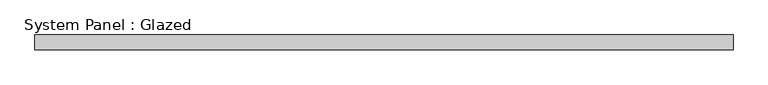
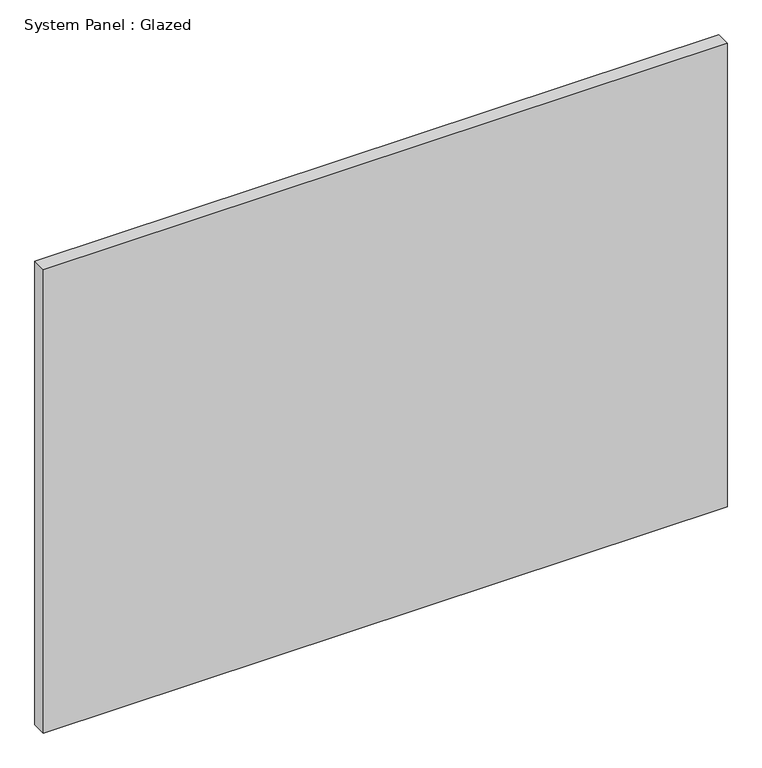
"""IFC4 building model written with IfcOpenShell, lengths in millimetres: plate geometry, System Panel : Glazed."""

from ifc_helpers import new_model, si_unit, origin, origin_with_axes, place, context, project, spatial, polyline, outline, extrude, source, transform, mapped, element, save


def system_panel_glazed_00a161e3(model_context):
    return source(origin(), model_context, "Body", "SweptSolid", [
        extrude(outline(polyline([(593.725, 19.05), (-593.725, 19.05), (-593.725, 44.45), (593.725, 44.45), (593.725, 19.05)])), origin_with_axes(), (0.0, 0.0, 1.0), 850.9),
    ])


if __name__ == "__main__":
    model = new_model("IFC4")
    model_context = context("Model", 3, world=origin())
    ifc_project = project(units=[si_unit("LENGTHUNIT", "METRE", prefix="MILLI")], contexts=[model_context])
    site = spatial("IfcSite", under=ifc_project)
    building = spatial("IfcBuilding", under=site)
    placement = place(None, origin())
    system_panel_glazed_shape = system_panel_glazed_00a161e3(model_context)
    element("IfcPlate", 1, ObjectType="System Panel : Glazed", at=placement, inside=building, context=model_context, shape_type="MappedRepresentation", body=[
        mapped(system_panel_glazed_shape, transform((0.0, 0.0, 0.0), x_axis=(1.0, 0.0, 0.0), y_axis=(0.0, 1.0, 0.0), z_axis=(0.0, 0.0, 1.0))),
    ])
    save(model, "model.ifc")

# Revit data of these elements
# Type "System Panel : Glazed"
#   Construction Type Id = "GSP4R"
#   Analytic Construction = "1/8 in Pilkington single glazing"
#   Visual Light Transmittance = 0.9
#   Solar Heat Gain Coefficient = 0.86
#   Heat Transfer Coefficient (U) = 1.18115 BTU/(h·ft²·°F)
#   Define Thermal Properties by = 1
# Element 1 (IfcPlate, "System Panel : Glazed")
#   Materials on its faces: "Glass"
# Materials
#   "Glass": class "Glass", colour RGB 0 128 192, transparency 0.75, Description = "Soda Lime Glass", Cost = 0
